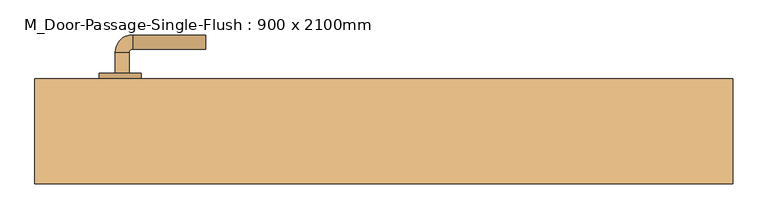
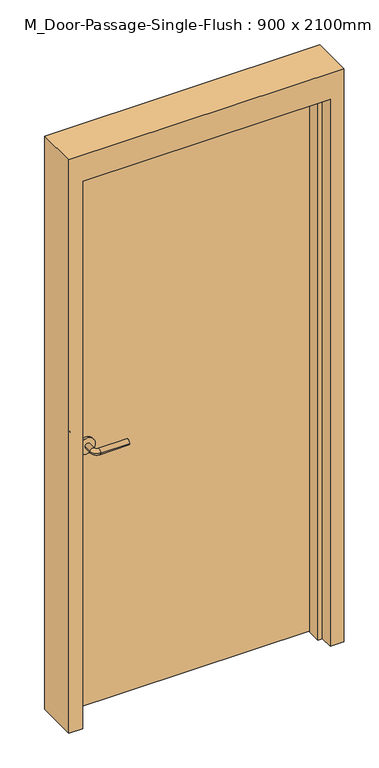
"""IFC4 building model written with IfcOpenShell, lengths in millimetres: door geometry, M_Door-Passage-Single-Flush : 900 x 2100mm."""

import ifcopenshell
import ifcopenshell.guid

model = None  # the IFC model being written
_history = None  # IfcOwnerHistory: only IFC2X3 demands one
_inside = {}  # id of a spatial element -> (the spatial element, [elements in it])
_under = {}  # id of a project, library or spatial element -> (it, [spatial elements below it])
_declared = {}  # id of a project -> (the project, [libraries it declares])
_typed = {}  # id of a type object -> (the type object, [elements of that type])
_made_of = {}  # id of a material, layer set ... -> (it, [elements and type objects made of it])


def new_model(schema):
    """Start an empty IFC model of exactly this schema.

    Asked for "IFC4X3", IfcOpenShell would pick the latest addendum, in which some entities
    have other attributes; the version numbers below select the first issue.
    IFC2X3 requires an IfcOwnerHistory on every rooted entity: one is made here for all.
    """
    global model, _history
    if schema == "IFC4X3":
        model = ifcopenshell.file(schema_version=(4, 3, 0, 0))
    else:
        model = ifcopenshell.file(schema=schema)
    _inside.clear()
    _under.clear()
    _declared.clear()
    _typed.clear()
    _made_of.clear()
    _history = None
    if model.schema == "IFC2X3":
        org = make("IfcOrganization", Name="unknown")
        user = make(
            "IfcPersonAndOrganization",
            ThePerson=make("IfcPerson", FamilyName="unknown"),
            TheOrganization=org,
        )
        app = make(
            "IfcApplication",
            ApplicationDeveloper=org,
            Version="unknown",
            ApplicationFullName="unknown",
            ApplicationIdentifier="unknown",
        )
        _history = make(
            "IfcOwnerHistory",
            OwningUser=user,
            OwningApplication=app,
            ChangeAction="ADDED",
            CreationDate=0,
        )
    return model


def make(cls, **values):
    """One entity of the class cls with the attributes given. An attribute that is None is left unset."""
    return model.create_entity(
        cls, **{name: value for name, value in values.items() if value is not None}
    )


def rooted(cls, **values):
    """An entity with a GlobalId (a new one), such as an element, a storey or a relation."""
    return make(cls, GlobalId=ifcopenshell.guid.new(), OwnerHistory=_history, **values)


def si_unit(unit_type, name, prefix=None):
    """IfcSIUnit, for example si_unit("LENGTHUNIT", "METRE", prefix="MILLI")."""
    return make("IfcSIUnit", UnitType=unit_type, Prefix=prefix, Name=name)


def assignment(units):
    """IfcUnitAssignment: the units of a project."""
    return None if units is None else make("IfcUnitAssignment", Units=units)


def point(xyz):
    """IfcCartesianPoint."""
    return None if xyz is None else make("IfcCartesianPoint", Coordinates=xyz)


def direction(xyz):
    """IfcDirection."""
    return None if xyz is None else make("IfcDirection", DirectionRatios=xyz)


def frame(location, z_axis=None, x_axis=None):
    """IfcAxis2Placement3D, a coordinate frame: its origin and axes. An axis left out is left unset."""
    return make(
        "IfcAxis2Placement3D",
        Location=point(location),
        Axis=direction(z_axis),
        RefDirection=direction(x_axis),
    )


def frame_2d(location, x_axis=None):
    """IfcAxis2Placement2D, a coordinate frame in the plane: its origin and x axis."""
    return make(
        "IfcAxis2Placement2D", Location=point(location), RefDirection=direction(x_axis)
    )


def origin():
    """The frame at (0, 0, 0) with its axes left unset."""
    return frame((0.0, 0.0, 0.0))


def origin_with_axes():
    """The frame at (0, 0, 0) with the z axis (0, 0, 1) and the x axis (1, 0, 0) written out."""
    return frame((0.0, 0.0, 0.0), z_axis=(0.0, 0.0, 1.0), x_axis=(1.0, 0.0, 0.0))


def place(relative_to, where):
    """IfcLocalPlacement: puts the frame where relative to a parent placement (None: the world)."""
    return make(
        "IfcLocalPlacement", PlacementRelTo=relative_to, RelativePlacement=where
    )


def context(
    kind, dimensions, precision=None, world=None, true_north=None, identifier=None
):
    """IfcGeometricRepresentationContext, for example the 3D "Model" context."""
    return make(
        "IfcGeometricRepresentationContext",
        ContextIdentifier=identifier,
        ContextType=kind,
        CoordinateSpaceDimension=dimensions,
        Precision=precision,
        WorldCoordinateSystem=world,
        TrueNorth=true_north,
    )


def project(units=None, contexts=None):
    """IfcProject with its units and contexts."""
    return rooted(
        "IfcProject",
        Name="project",
        RepresentationContexts=contexts,
        UnitsInContext=assignment(units),
    )


def spatial(cls, under=None, at=None, **own):
    """A site, building, storey or space (cls), placed at a placement, below another one or the project."""
    s = rooted(cls, ObjectPlacement=at, **own)
    if under is not None:
        _under.setdefault(under.id(), (under, []))[1].append(s)
    return s


def polyline(points):
    """IfcPolyline through the points."""
    return make("IfcPolyline", Points=[point(p) for p in points])


def circle_curve(where, radius):
    """IfcCircle in the frame where."""
    return make("IfcCircle", Position=where, Radius=radius)


def ellipse_curve(where, semi_axis1, semi_axis2):
    """IfcEllipse in the frame where."""
    return make(
        "IfcEllipse", Position=where, SemiAxis1=semi_axis1, SemiAxis2=semi_axis2
    )


def trimmed(basis, trim1, trim2, sense, master):
    """IfcTrimmedCurve: the piece of a basis curve between two trims."""
    return make(
        "IfcTrimmedCurve",
        BasisCurve=basis,
        Trim1=trim1,
        Trim2=trim2,
        SenseAgreement=sense,
        MasterRepresentation=master,
    )


def segment(curve, same_sense, transition):
    """IfcCompositeCurveSegment."""
    return make(
        "IfcCompositeCurveSegment",
        Transition=transition,
        SameSense=same_sense,
        ParentCurve=curve,
    )


def composite_curve(segments, self_intersect=None):
    """IfcCompositeCurve: segments joined end to end."""
    return make("IfcCompositeCurve", Segments=segments, SelfIntersect=self_intersect)


def outline(outer, holes=None, kind="AREA"):
    """IfcArbitraryClosedProfileDef: a profile drawn as a closed curve; with holes, ...WithVoids."""
    if holes is None:
        return make("IfcArbitraryClosedProfileDef", ProfileType=kind, OuterCurve=outer)
    return make(
        "IfcArbitraryProfileDefWithVoids",
        ProfileType=kind,
        OuterCurve=outer,
        InnerCurves=holes,
    )


def extrude(swept, where, along, depth):
    """IfcExtrudedAreaSolid: the profile swept, set in the frame where, extruded along a direction by depth."""
    return make(
        "IfcExtrudedAreaSolid",
        SweptArea=swept,
        Position=where,
        ExtrudedDirection=direction(along),
        Depth=depth,
    )


def faces_of(points, faces, orient=None, outer=None):
    """IfcFace entities. A face is a list of loops; a loop is a list of indices into points, from 0.

    orient and outer hold one flag for each loop. By default every Orientation is true, the
    first loop of a face is its IfcFaceOuterBound and the others are IfcFaceBound.
    """
    made = []
    for i, loops in enumerate(faces):
        bounds = []
        for j, loop in enumerate(loops):
            is_outer = j == 0 if outer is None else outer[i][j]
            bounds.append(
                make(
                    "IfcFaceOuterBound" if is_outer else "IfcFaceBound",
                    Bound=make("IfcPolyLoop", Polygon=[points[k] for k in loop]),
                    Orientation=True if orient is None else orient[i][j],
                )
            )
        made.append(make("IfcFace", Bounds=bounds))
    return made


def faceted_brep(points, faces, orient=None, outer=None, voids=None):
    """IfcFacetedBrep: a solid bounded by flat faces; with voids (closed shells), ...WithVoids."""
    shared = [point(p) for p in points]
    hull = make("IfcClosedShell", CfsFaces=faces_of(shared, faces, orient, outer))
    if voids is None:
        return make("IfcFacetedBrep", Outer=hull)
    return make(
        "IfcFacetedBrepWithVoids",
        Outer=hull,
        Voids=[
            make(cls, CfsFaces=faces_of(shared, fs, o, b)) for cls, fs, o, b in voids
        ],
    )


def shape(context_of_items, identifier, shape_type, items):
    """IfcShapeRepresentation: the items that make up one representation, for example the "Body"."""
    return make(
        "IfcShapeRepresentation",
        ContextOfItems=context_of_items,
        RepresentationIdentifier=identifier,
        RepresentationType=shape_type,
        Items=items,
    )


def source(mapping_origin, context_of_items, identifier, shape_type, items):
    """IfcRepresentationMap: a shape defined once, which mapped items show again and again."""
    return make(
        "IfcRepresentationMap",
        MappingOrigin=mapping_origin,
        MappedRepresentation=shape(context_of_items, identifier, shape_type, items),
    )


def transform(
    local_origin,
    x_axis=None,
    y_axis=None,
    z_axis=None,
    scale=None,
    scale2=None,
    scale3=None,
    uniform=True,
):
    """IfcCartesianTransformationOperator3D, or its non-uniform kind. x_axis, y_axis, z_axis: its Axis1, 2, 3."""
    if uniform:
        return make(
            "IfcCartesianTransformationOperator3D",
            Axis1=direction(x_axis),
            Axis2=direction(y_axis),
            LocalOrigin=point(local_origin),
            Scale=scale,
            Axis3=direction(z_axis),
        )
    return make(
        "IfcCartesianTransformationOperator3DnonUniform",
        Axis1=direction(x_axis),
        Axis2=direction(y_axis),
        LocalOrigin=point(local_origin),
        Scale=scale,
        Axis3=direction(z_axis),
        Scale2=scale2,
        Scale3=scale3,
    )


def mapped(mapping_source, mapping_target):
    """IfcMappedItem: shows the shape of a source again, moved by a transform."""
    return make(
        "IfcMappedItem", MappingSource=mapping_source, MappingTarget=mapping_target
    )


def made_of(thing, what):
    """Note that an element or type object is made of a material, layer set ...; save() writes the relation."""
    if what is not None:
        _made_of.setdefault(what.id(), (what, []))[1].append(thing)
    return thing


def element(
    cls,
    number,
    at=None,
    inside=None,
    cuts=None,
    type_object=None,
    material=None,
    context=None,
    identifier="Body",
    shape_type=None,
    held_by="IfcProductDefinitionShape",
    body=None,
    shapes=None,
    **own,
):
    """One element of the class cls, such as IfcWall. Its Tag is "e" and its number.

    at: its placement. inside: the storey or other place that contains it. cuts: it is an
    opening in that element (IfcRelVoidsElement). A single representation is given by context,
    identifier, shape_type and body (its items); several are given by shapes. held_by: the class
    of the entity that holds the representations. save() writes the other relations.
    """
    e = rooted(cls, Tag="e%d" % number, ObjectPlacement=at, **own)
    if body is not None:
        shapes = [shape(context, identifier, shape_type, body)]
    if shapes is not None:
        e.Representation = make(held_by, Representations=shapes)
    if inside is not None:
        _inside.setdefault(inside.id(), (inside, []))[1].append(e)
    if cuts is not None:
        rooted(
            "IfcRelVoidsElement", RelatingBuildingElement=cuts, RelatedOpeningElement=e
        )
    if type_object is not None:
        _typed.setdefault(type_object.id(), (type_object, []))[1].append(e)
    return made_of(e, material)


def aggregate(whole, parts):
    """IfcRelAggregates: a whole, such as a stair, and the parts it consists of."""
    return rooted("IfcRelAggregates", RelatingObject=whole, RelatedObjects=parts)


def save(model, path):
    """Write the relations noted so far, then the file.

    IfcRelAggregates (storeys below a building ...), IfcRelContainedInSpatialStructure (elements
    in a storey), IfcRelDefinesByType, IfcRelAssociatesMaterial and IfcRelDeclares: one each for
    every whole, place, type object, material and project.
    """
    for whole, parts in _under.values():
        aggregate(whole, parts)
    for where, things in _inside.values():
        rooted(
            "IfcRelContainedInSpatialStructure",
            RelatedElements=things,
            RelatingStructure=where,
        )
    for kind, things in _typed.values():
        rooted("IfcRelDefinesByType", RelatedObjects=things, RelatingType=kind)
    for what, things in _made_of.values():
        rooted("IfcRelAssociatesMaterial", RelatedObjects=things, RelatingMaterial=what)
    for by, libraries in _declared.values():
        rooted("IfcRelDeclares", RelatingContext=by, RelatedDefinitions=libraries)
    model.write(path)


def plane_surface(at):
    """IfcPlane: the flat surface through the origin of the frame at, square to its z axis."""
    return make("IfcPlane", Position=at)


def cylinder_surface(at, radius):
    """IfcCylindricalSurface: all points at the distance radius from the z axis of the frame at."""
    return make("IfcCylindricalSurface", Position=at, Radius=radius)


def revolved_surface(curve, axis_point, axis_direction):
    """IfcSurfaceOfRevolution: the curve turned about the line through axis_point along axis_direction."""
    return make(
        "IfcSurfaceOfRevolution",
        SweptCurve=make("IfcArbitraryOpenProfileDef", ProfileType="CURVE", Curve=curve),
        AxisPosition=make("IfcAxis1Placement", Location=point(axis_point), Axis=direction(axis_direction)),
    )


def advanced_brep(points, edges, surfaces, faces):
    """IfcAdvancedBrep: a solid bounded by faces that lie on surfaces and meet in shared edges.

    An edge is (start, end): straight between two places in points (the first is 0);
    or (start, end, curve); or (start, end, curve, False) where it runs against its curve.
    A face is (place in surfaces, loops), or (place, loops, False) where it looks against
    its surface's normal. A loop lists edges by number (the first is 1), with a minus sign
    where the edge is run from its end to its start. The first loop is the outer one.
    """
    corners = [point(p) for p in points]
    vertices = [make("IfcVertexPoint", VertexGeometry=c) for c in corners]
    made = []
    for start, end, *more in edges:
        made.append(
            make(
                "IfcEdgeCurve",
                EdgeStart=vertices[start],
                EdgeEnd=vertices[end],
                EdgeGeometry=more[0] if more else make("IfcPolyline", Points=[corners[start], corners[end]]),
                SameSense=more[1] if len(more) > 1 else True,
            )
        )
    hull = []
    for where, loops, *sense in faces:
        bounds = []
        for j, loop in enumerate(loops):
            ring = [make("IfcOrientedEdge", EdgeElement=made[abs(k) - 1], Orientation=k > 0) for k in loop]
            bounds.append(
                make(
                    "IfcFaceOuterBound" if j == 0 else "IfcFaceBound",
                    Bound=make("IfcEdgeLoop", EdgeList=ring),
                    Orientation=True,
                )
            )
        hull.append(make("IfcAdvancedFace", Bounds=bounds, FaceSurface=surfaces[where], SameSense=sense[0] if sense else True))
    return make("IfcAdvancedBrep", Outer=make("IfcClosedShell", CfsFaces=hull))


def m_door_passage_single_flush_900_x_2100mm_f70d95c9(model_context):
    return source(origin(), model_context, "Body", "SolidModel", [
        advanced_brep(
        [(-384.990625, 3.35, 1000.0), (-364.990625, 3.35, 1000.0), (-364.990625, -26.65, 1000.0), (-384.990625, -26.65, 1000.0), (-359.990625, -31.65, 1000.0), (-359.990625, -51.65, 1000.0), (-254.990625, -51.65, 1000.0), (-254.990625, -31.65, 1000.0)],
        [
            (0, 1, circle_curve(frame((-374.990625, 3.35, 1000.0), z_axis=(0.0, 1.0, 0.0), x_axis=(1.0, 0.0, 0.0)), 10.0)),
            (1, 0, circle_curve(frame((-374.990625, 3.35, 1000.0), z_axis=(0.0, 1.0, 0.0), x_axis=(1.0, 0.0, 0.0)), 10.0)),
            (1, 2),
            (2, 3, circle_curve(frame((-374.990625, -26.65, 1000.0), z_axis=(0.0, 1.0, 0.0), x_axis=(1.0, 0.0, 0.0)), 10.0)),
            (3, 0),
            (3, 2, circle_curve(frame((-374.990625, -26.65, 1000.0), z_axis=(0.0, 1.0, 0.0), x_axis=(1.0, 0.0, 0.0)), 10.0)),
            (4, 5, circle_curve(frame((-359.990625, -41.65, 1000.0), z_axis=(-1.0, 0.0, 0.0), x_axis=(0.0, 1.0, 0.0)), 10.0)),
            (5, 3, circle_curve(frame((-359.990625, -26.65, 1000.0), z_axis=(0.0, 0.0, -1.0), x_axis=(-1.0, 0.0, 0.0)), 25.0)),
            (2, 4, circle_curve(frame((-359.990625, -26.65, 1000.0), z_axis=(0.0, 0.0, 1.0), x_axis=(-1.0, 0.0, 0.0)), 5.0)),
            (5, 4, circle_curve(frame((-359.990625, -41.65, 1000.0), z_axis=(-1.0, 0.0, 0.0), x_axis=(0.0, 1.0, 0.0)), 10.0)),
            (6, 7, circle_curve(frame((-254.990625, -41.65, 1000.0), z_axis=(1.0, 0.0, 0.0), x_axis=(0.0, 1.0, 0.0)), 10.0)),
            (7, 6, circle_curve(frame((-254.990625, -41.65, 1000.0), z_axis=(1.0, 0.0, 0.0), x_axis=(0.0, 1.0, 0.0)), 10.0)),
            (4, 7),
            (6, 5),
        ],
        [
            plane_surface(frame((-374.990625, 3.35, 1000.0), z_axis=(0.0, 1.0, 0.0), x_axis=(0.0, 0.0, 1.0))),
            cylinder_surface(frame((-374.990625, 3.35, 1000.0), z_axis=(0.0, 1.0, 0.0), x_axis=(1.0, 0.0, 0.0)), 10.0),
            revolved_surface(trimmed(ellipse_curve(frame((-374.990625, -26.65, 1000.0), z_axis=(0.0, -1.0, 0.0), x_axis=(1.0, 0.0, 0.0)), 10.0, 10.0), [point((-384.990625, -26.65, 1000.0))], [point((-364.990625, -26.65, 1000.0))], True, "CARTESIAN"), (-359.990625, -26.65, 1000.0), (0.0, 0.0, -1.0)),
            revolved_surface(trimmed(ellipse_curve(frame((-374.990625, -26.65, 1000.0), z_axis=(0.0, -1.0, 0.0), x_axis=(1.0, 0.0, 0.0)), 10.0, 10.0), [point((-364.990625, -26.65, 1000.0))], [point((-384.990625, -26.65, 1000.0))], True, "CARTESIAN"), (-359.990625, -26.65, 1000.0), (0.0, 0.0, -1.0)),
            plane_surface(frame((-254.990625, -41.65, 1000.0), z_axis=(1.0, 0.0, 0.0), x_axis=(0.0, 0.0, 1.0))),
            cylinder_surface(frame((-359.990625, -41.65, 1000.0), z_axis=(-1.0, 0.0, 0.0), x_axis=(0.0, 1.0, 0.0)), 10.0),
        ],
        [
            (0, [[1, 2]]),
            (1, [[3, 4, 5, -2]]),
            (1, [[-5, 6, -3, -1]]),
            (2, [[7, 8, -4, 9]]),
            (3, [[10, -9, -6, -8]]),
            (4, [[11, 12]]),
            (5, [[13, -11, 14, -7]]),
            (5, [[-14, -12, -13, -10]]),
        ],
    ),
        extrude(outline(composite_curve([segment(trimmed(circle_curve(frame_2d((1000.0, -377.490625)), 30.0), [point((1000.0, -407.490625))], [point((1000.0, -347.490625))], False, "CARTESIAN"), True, "CONTINUOUS"), segment(trimmed(circle_curve(frame_2d((1000.0, -377.490625)), 30.0), [point((1000.0, -347.490625))], [point((1000.0, -407.490625))], False, "CARTESIAN"), True, "CONTINUOUS")], self_intersect=False)), frame((0.0, 3.35, 0.0), z_axis=(0.0, 1.0, 0.0), x_axis=(0.0, 0.0, 1.0)), (0.0, 0.0, 1.0), 8.0),
        advanced_brep(
        [(-384.990625, 64.35, 1000.0), (-364.990625, 64.35, 1000.0), (-384.990625, 94.35, 1000.0), (-364.990625, 94.35, 1000.0), (-359.990625, 99.35, 1000.0), (-359.990625, 119.35, 1000.0), (-254.990625, 119.35, 1000.0), (-254.990625, 99.35, 1000.0)],
        [
            (0, 1, circle_curve(frame((-374.990625, 64.35, 1000.0), z_axis=(0.0, -1.0, 0.0), x_axis=(1.0, 0.0, 0.0)), 10.0)),
            (1, 0, circle_curve(frame((-374.990625, 64.35, 1000.0), z_axis=(0.0, -1.0, 0.0), x_axis=(1.0, 0.0, 0.0)), 10.0)),
            (0, 2),
            (2, 3, circle_curve(frame((-374.990625, 94.35, 1000.0), z_axis=(0.0, -1.0, 0.0), x_axis=(1.0, 0.0, 0.0)), 10.0)),
            (3, 1),
            (3, 2, circle_curve(frame((-374.990625, 94.35, 1000.0), z_axis=(0.0, -1.0, 0.0), x_axis=(1.0, 0.0, 0.0)), 10.0)),
            (4, 3, circle_curve(frame((-359.990625, 94.35, 1000.0), z_axis=(0.0, 0.0, 1.0), x_axis=(-1.0, 0.0, 0.0)), 5.0)),
            (2, 5, circle_curve(frame((-359.990625, 94.35, 1000.0), z_axis=(0.0, 0.0, -1.0), x_axis=(-1.0, 0.0, 0.0)), 25.0)),
            (5, 4, circle_curve(frame((-359.990625, 109.35, 1000.0), z_axis=(-1.0, 0.0, 0.0), x_axis=(0.0, -1.0, 0.0)), 10.0)),
            (4, 5, circle_curve(frame((-359.990625, 109.35, 1000.0), z_axis=(-1.0, 0.0, 0.0), x_axis=(0.0, -1.0, 0.0)), 10.0)),
            (6, 7, circle_curve(frame((-254.990625, 109.35, 1000.0), z_axis=(1.0, 0.0, 0.0), x_axis=(0.0, -1.0, 0.0)), 10.0)),
            (7, 6, circle_curve(frame((-254.990625, 109.35, 1000.0), z_axis=(1.0, 0.0, 0.0), x_axis=(0.0, -1.0, 0.0)), 10.0)),
            (5, 6),
            (7, 4),
        ],
        [
            plane_surface(frame((-374.990625, 64.35, 1000.0), z_axis=(0.0, -1.0, 0.0), x_axis=(0.0, 0.0, 1.0))),
            cylinder_surface(frame((-374.990625, 64.35, 1000.0), z_axis=(0.0, -1.0, 0.0), x_axis=(1.0, 0.0, 0.0)), 10.0),
            revolved_surface(trimmed(ellipse_curve(frame((-374.990625, 94.35, 1000.0), z_axis=(0.0, -1.0, 0.0), x_axis=(1.0, 0.0, 0.0)), 10.0, 10.0), [point((-384.990625, 94.35, 1000.0))], [point((-364.990625, 94.35, 1000.0))], True, "CARTESIAN"), (-359.990625, 94.35, 1000.0), (0.0, 0.0, -1.0)),
            revolved_surface(trimmed(ellipse_curve(frame((-374.990625, 94.35, 1000.0), z_axis=(0.0, -1.0, 0.0), x_axis=(1.0, 0.0, 0.0)), 10.0, 10.0), [point((-364.990625, 94.35, 1000.0))], [point((-384.990625, 94.35, 1000.0))], True, "CARTESIAN"), (-359.990625, 94.35, 1000.0), (0.0, 0.0, -1.0)),
            plane_surface(frame((-254.990625, 109.35, 1000.0), z_axis=(1.0, 0.0, 0.0), x_axis=(0.0, 0.0, 1.0))),
            cylinder_surface(frame((-359.990625, 109.35, 1000.0), z_axis=(-1.0, 0.0, 0.0), x_axis=(0.0, -1.0, 0.0)), 10.0),
        ],
        [
            (0, [[1, 2]]),
            (1, [[-1, 3, 4, 5]]),
            (1, [[-2, -5, 6, -3]]),
            (2, [[7, -4, 8, 9]]),
            (3, [[-8, -6, -7, 10]]),
            (4, [[11, 12]]),
            (5, [[-9, 13, -12, 14]]),
            (5, [[-10, -14, -11, -13]]),
        ],
    ),
        extrude(outline(composite_curve([segment(trimmed(circle_curve(frame_2d((1000.0, -377.490625)), 30.0), [point((1000.0, -407.490625))], [point((1000.0, -347.490625))], False, "CARTESIAN"), True, "CONTINUOUS"), segment(trimmed(circle_curve(frame_2d((1000.0, -377.490625)), 30.0), [point((1000.0, -347.490625))], [point((1000.0, -407.490625))], False, "CARTESIAN"), True, "CONTINUOUS")], self_intersect=False)), frame((0.0, 56.35, 0.0), z_axis=(0.0, 1.0, 0.0), x_axis=(0.0, 0.0, 1.0)), (0.0, 0.0, 1.0), 8.0),
        extrude(outline(polyline([(450.0, 11.35), (-450.0, 11.35), (-450.0, 56.35), (450.0, 56.35), (450.0, 11.35)])), origin_with_axes(), (0.0, 0.0, 1.0), 2100.0),
        faceted_brep([(450.0, 6.5875, 0.0), (450.0, 56.35, 0.0), (500.0, 56.35, 0.0), (500.0, -93.65, 0.0), (450.0, -93.65, 0.0), (450.0, -44.4375, 0.0), (434.125, -44.4375, 0.0), (434.125, 6.5875, 0.0), (450.0, 6.5875, 2100.0), (450.0, 56.35, 2100.0), (-450.0, 56.35, 2100.0), (-450.0, 56.35, 0.0), (-500.0, 56.35, 0.0), (-500.0, 56.35, 2200.0), (500.0, 56.35, 2200.0), (500.0, -93.65, 2200.0), (-500.0, -93.65, 2200.0), (-500.0, -93.65, 0.0), (-450.0, -93.65, 0.0), (-450.0, -93.65, 2100.0), (450.0, -93.65, 2100.0), (450.0, -44.4375, 2100.0), (-450.0, -44.4375, 2100.0), (-450.0, -44.4375, 0.0), (-434.125, -44.4375, 0.0), (-434.125, -44.4375, 2084.125), (434.125, -44.4375, 2084.125), (434.125, 6.5875, 2084.125), (-434.125, 6.5875, 2084.125), (-434.125, 6.5875, 0.0), (-450.0, 6.5875, 0.0), (-450.0, 6.5875, 2100.0)], [[[0, 1, 2, 3, 4, 5, 6, 7]], [[1, 0, 8, 9]], [[2, 1, 9, 10, 11, 12, 13, 14]], [[3, 2, 14, 15]], [[4, 3, 15, 16, 17, 18, 19, 20]], [[5, 4, 20, 21]], [[6, 5, 21, 22, 23, 24, 25, 26]], [[7, 6, 26, 27]], [[0, 7, 27, 28, 29, 30, 31, 8]], [[9, 8, 31, 10]], [[20, 19, 22, 21]], [[26, 25, 28, 27]], [[12, 11, 30, 29, 24, 23, 18, 17]], [[11, 10, 31, 30]], [[13, 12, 17, 16]], [[19, 18, 23, 22]], [[25, 24, 29, 28]], [[15, 14, 13, 16]]]),
    ])


if __name__ == "__main__":
    model = new_model("IFC4")
    model_context = context("Model", 3, world=origin())
    ifc_project = project(units=[si_unit("LENGTHUNIT", "METRE", prefix="MILLI")], contexts=[model_context])
    site = spatial("IfcSite", under=ifc_project)
    building = spatial("IfcBuilding", under=site)
    placement = place(None, origin())
    m_door_passage_single_flush_900_x_2100mm_shape = m_door_passage_single_flush_900_x_2100mm_f70d95c9(model_context)
    element("IfcDoor", 1, ObjectType="M_Door-Passage-Single-Flush : 900 x 2100mm", at=placement, inside=building, context=model_context, shape_type="MappedRepresentation", body=[
        mapped(m_door_passage_single_flush_900_x_2100mm_shape, transform((0.0, 0.0, 0.0), x_axis=(1.0, 0.0, 0.0), y_axis=(0.0, 1.0, 0.0), z_axis=(0.0, 0.0, 1.0))),
    ])
    save(model, "model.ifc")

# Revit data of these elements
# Type "M_Door-Passage-Single-Flush : 900 x 2100mm"
#   Type Mark = "38"
#   Analytic Construction = "Wooden"
#   Thickness = 45 mm
#   Thermal Resistance (R) = 0.455703 (m²·K)/W
#   Swing Angle [instance default] = 90.00°
#   Strike Height = 1000 mm
#   Rough Width [instance default] = 1000 mm
#   Rough Height [instance default] = 2200 mm
#   MF Opening Height [instance default] = 100 mm
#   MF Opening Width [instance default] = 100 mm
#   Inset Calculate [instance default] = 105 mm
#   Masonry Inset [instance default] = 25 mm
#   Height = 2100 mm
#   Width = 900 mm
#   Heat Transfer Coefficient (U) = 2.19465 W/(m²·K)
#   Masonry Frame Depth = 150 mm
#   Masonry Frame [instance default] = yes
#   Function = 1
#   Dry Wall Frame [instance default] = no
#   Panel Material = Wood - Birch
#   Frame Material = Metal - Paint Finish - Grey
#   Door Handle Material = Aluminum
#   Visual Light Transmittance = 0
#   Solar Heat Gain Coefficient = 0
#   Wall Closure = (empty or 0)
# Element 1 (IfcDoor, "M_Door-Passage-Single-Flush : 900 x 2100mm")
#   Materials on its faces: "Aluminum", "Metal - Paint Finish - Grey", "Wood - Birch"
# Materials
#   "Wood - Birch": class "Wood", colour RGB 173 132 96, transparency 0, Cost = 0
#   "Metal - Paint Finish - Grey": class "Paint", colour RGB 178 178 178, transparency 0, Cost = 0
#   "Aluminum": class "Metal", colour RGB 244 245 246, transparency 0, Description = "Aluminum 6061", Cost = 0
